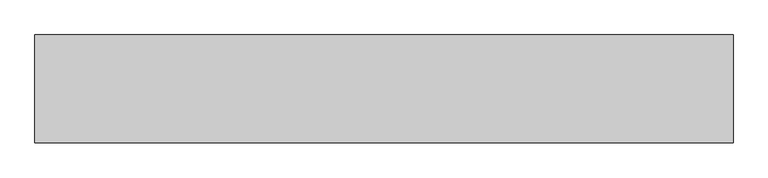
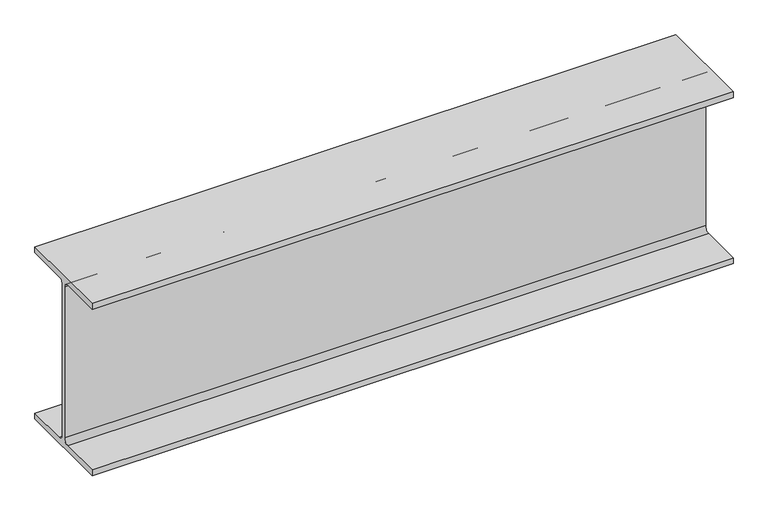
"""IFC4 building model written with IfcOpenShell, lengths in millimetres: beam geometry, Old_Steel Beam_H-KSD3502 : H_SB_ASB_H-194×150x6x9."""

import ifcopenshell
import ifcopenshell.guid

model = None  # the IFC model being written
_history = None  # IfcOwnerHistory: only IFC2X3 demands one
_inside = {}  # id of a spatial element -> (the spatial element, [elements in it])
_under = {}  # id of a project, library or spatial element -> (it, [spatial elements below it])
_declared = {}  # id of a project -> (the project, [libraries it declares])
_typed = {}  # id of a type object -> (the type object, [elements of that type])
_made_of = {}  # id of a material, layer set ... -> (it, [elements and type objects made of it])


def new_model(schema):
    """Start an empty IFC model of exactly this schema.

    Asked for "IFC4X3", IfcOpenShell would pick the latest addendum, in which some entities
    have other attributes; the version numbers below select the first issue.
    IFC2X3 requires an IfcOwnerHistory on every rooted entity: one is made here for all.
    """
    global model, _history
    if schema == "IFC4X3":
        model = ifcopenshell.file(schema_version=(4, 3, 0, 0))
    else:
        model = ifcopenshell.file(schema=schema)
    _inside.clear()
    _under.clear()
    _declared.clear()
    _typed.clear()
    _made_of.clear()
    _history = None
    if model.schema == "IFC2X3":
        org = make("IfcOrganization", Name="unknown")
        user = make(
            "IfcPersonAndOrganization",
            ThePerson=make("IfcPerson", FamilyName="unknown"),
            TheOrganization=org,
        )
        app = make(
            "IfcApplication",
            ApplicationDeveloper=org,
            Version="unknown",
            ApplicationFullName="unknown",
            ApplicationIdentifier="unknown",
        )
        _history = make(
            "IfcOwnerHistory",
            OwningUser=user,
            OwningApplication=app,
            ChangeAction="ADDED",
            CreationDate=0,
        )
    return model


def make(cls, **values):
    """One entity of the class cls with the attributes given. An attribute that is None is left unset."""
    return model.create_entity(
        cls, **{name: value for name, value in values.items() if value is not None}
    )


def rooted(cls, **values):
    """An entity with a GlobalId (a new one), such as an element, a storey or a relation."""
    return make(cls, GlobalId=ifcopenshell.guid.new(), OwnerHistory=_history, **values)


def si_unit(unit_type, name, prefix=None):
    """IfcSIUnit, for example si_unit("LENGTHUNIT", "METRE", prefix="MILLI")."""
    return make("IfcSIUnit", UnitType=unit_type, Prefix=prefix, Name=name)


def assignment(units):
    """IfcUnitAssignment: the units of a project."""
    return None if units is None else make("IfcUnitAssignment", Units=units)


def point(xyz):
    """IfcCartesianPoint."""
    return None if xyz is None else make("IfcCartesianPoint", Coordinates=xyz)


def direction(xyz):
    """IfcDirection."""
    return None if xyz is None else make("IfcDirection", DirectionRatios=xyz)


def frame(location, z_axis=None, x_axis=None):
    """IfcAxis2Placement3D, a coordinate frame: its origin and axes. An axis left out is left unset."""
    return make(
        "IfcAxis2Placement3D",
        Location=point(location),
        Axis=direction(z_axis),
        RefDirection=direction(x_axis),
    )


def frame_2d(location, x_axis=None):
    """IfcAxis2Placement2D, a coordinate frame in the plane: its origin and x axis."""
    return make(
        "IfcAxis2Placement2D", Location=point(location), RefDirection=direction(x_axis)
    )


def origin():
    """The frame at (0, 0, 0) with its axes left unset."""
    return frame((0.0, 0.0, 0.0))


def place(relative_to, where):
    """IfcLocalPlacement: puts the frame where relative to a parent placement (None: the world)."""
    return make(
        "IfcLocalPlacement", PlacementRelTo=relative_to, RelativePlacement=where
    )


def context(
    kind, dimensions, precision=None, world=None, true_north=None, identifier=None
):
    """IfcGeometricRepresentationContext, for example the 3D "Model" context."""
    return make(
        "IfcGeometricRepresentationContext",
        ContextIdentifier=identifier,
        ContextType=kind,
        CoordinateSpaceDimension=dimensions,
        Precision=precision,
        WorldCoordinateSystem=world,
        TrueNorth=true_north,
    )


def project(units=None, contexts=None):
    """IfcProject with its units and contexts."""
    return rooted(
        "IfcProject",
        Name="project",
        RepresentationContexts=contexts,
        UnitsInContext=assignment(units),
    )


def spatial(cls, under=None, at=None, **own):
    """A site, building, storey or space (cls), placed at a placement, below another one or the project."""
    s = rooted(cls, ObjectPlacement=at, **own)
    if under is not None:
        _under.setdefault(under.id(), (under, []))[1].append(s)
    return s


def polyline(points):
    """IfcPolyline through the points."""
    return make("IfcPolyline", Points=[point(p) for p in points])


def circle_curve(where, radius):
    """IfcCircle in the frame where."""
    return make("IfcCircle", Position=where, Radius=radius)


def trimmed(basis, trim1, trim2, sense, master):
    """IfcTrimmedCurve: the piece of a basis curve between two trims."""
    return make(
        "IfcTrimmedCurve",
        BasisCurve=basis,
        Trim1=trim1,
        Trim2=trim2,
        SenseAgreement=sense,
        MasterRepresentation=master,
    )


def segment(curve, same_sense, transition):
    """IfcCompositeCurveSegment."""
    return make(
        "IfcCompositeCurveSegment",
        Transition=transition,
        SameSense=same_sense,
        ParentCurve=curve,
    )


def composite_curve(segments, self_intersect=None):
    """IfcCompositeCurve: segments joined end to end."""
    return make("IfcCompositeCurve", Segments=segments, SelfIntersect=self_intersect)


def outline(outer, holes=None, kind="AREA"):
    """IfcArbitraryClosedProfileDef: a profile drawn as a closed curve; with holes, ...WithVoids."""
    if holes is None:
        return make("IfcArbitraryClosedProfileDef", ProfileType=kind, OuterCurve=outer)
    return make(
        "IfcArbitraryProfileDefWithVoids",
        ProfileType=kind,
        OuterCurve=outer,
        InnerCurves=holes,
    )


def extrude(swept, where, along, depth):
    """IfcExtrudedAreaSolid: the profile swept, set in the frame where, extruded along a direction by depth."""
    return make(
        "IfcExtrudedAreaSolid",
        SweptArea=swept,
        Position=where,
        ExtrudedDirection=direction(along),
        Depth=depth,
    )


def shape(context_of_items, identifier, shape_type, items):
    """IfcShapeRepresentation: the items that make up one representation, for example the "Body"."""
    return make(
        "IfcShapeRepresentation",
        ContextOfItems=context_of_items,
        RepresentationIdentifier=identifier,
        RepresentationType=shape_type,
        Items=items,
    )


def source(mapping_origin, context_of_items, identifier, shape_type, items):
    """IfcRepresentationMap: a shape defined once, which mapped items show again and again."""
    return make(
        "IfcRepresentationMap",
        MappingOrigin=mapping_origin,
        MappedRepresentation=shape(context_of_items, identifier, shape_type, items),
    )


def transform(
    local_origin,
    x_axis=None,
    y_axis=None,
    z_axis=None,
    scale=None,
    scale2=None,
    scale3=None,
    uniform=True,
):
    """IfcCartesianTransformationOperator3D, or its non-uniform kind. x_axis, y_axis, z_axis: its Axis1, 2, 3."""
    if uniform:
        return make(
            "IfcCartesianTransformationOperator3D",
            Axis1=direction(x_axis),
            Axis2=direction(y_axis),
            LocalOrigin=point(local_origin),
            Scale=scale,
            Axis3=direction(z_axis),
        )
    return make(
        "IfcCartesianTransformationOperator3DnonUniform",
        Axis1=direction(x_axis),
        Axis2=direction(y_axis),
        LocalOrigin=point(local_origin),
        Scale=scale,
        Axis3=direction(z_axis),
        Scale2=scale2,
        Scale3=scale3,
    )


def mapped(mapping_source, mapping_target):
    """IfcMappedItem: shows the shape of a source again, moved by a transform."""
    return make(
        "IfcMappedItem", MappingSource=mapping_source, MappingTarget=mapping_target
    )


def made_of(thing, what):
    """Note that an element or type object is made of a material, layer set ...; save() writes the relation."""
    if what is not None:
        _made_of.setdefault(what.id(), (what, []))[1].append(thing)
    return thing


def element(
    cls,
    number,
    at=None,
    inside=None,
    cuts=None,
    type_object=None,
    material=None,
    context=None,
    identifier="Body",
    shape_type=None,
    held_by="IfcProductDefinitionShape",
    body=None,
    shapes=None,
    **own,
):
    """One element of the class cls, such as IfcWall. Its Tag is "e" and its number.

    at: its placement. inside: the storey or other place that contains it. cuts: it is an
    opening in that element (IfcRelVoidsElement). A single representation is given by context,
    identifier, shape_type and body (its items); several are given by shapes. held_by: the class
    of the entity that holds the representations. save() writes the other relations.
    """
    e = rooted(cls, Tag="e%d" % number, ObjectPlacement=at, **own)
    if body is not None:
        shapes = [shape(context, identifier, shape_type, body)]
    if shapes is not None:
        e.Representation = make(held_by, Representations=shapes)
    if inside is not None:
        _inside.setdefault(inside.id(), (inside, []))[1].append(e)
    if cuts is not None:
        rooted(
            "IfcRelVoidsElement", RelatingBuildingElement=cuts, RelatedOpeningElement=e
        )
    if type_object is not None:
        _typed.setdefault(type_object.id(), (type_object, []))[1].append(e)
    return made_of(e, material)


def aggregate(whole, parts):
    """IfcRelAggregates: a whole, such as a stair, and the parts it consists of."""
    return rooted("IfcRelAggregates", RelatingObject=whole, RelatedObjects=parts)


def save(model, path):
    """Write the relations noted so far, then the file.

    IfcRelAggregates (storeys below a building ...), IfcRelContainedInSpatialStructure (elements
    in a storey), IfcRelDefinesByType, IfcRelAssociatesMaterial and IfcRelDeclares: one each for
    every whole, place, type object, material and project.
    """
    for whole, parts in _under.values():
        aggregate(whole, parts)
    for where, things in _inside.values():
        rooted(
            "IfcRelContainedInSpatialStructure",
            RelatedElements=things,
            RelatingStructure=where,
        )
    for kind, things in _typed.values():
        rooted("IfcRelDefinesByType", RelatedObjects=things, RelatingType=kind)
    for what, things in _made_of.values():
        rooted("IfcRelAssociatesMaterial", RelatedObjects=things, RelatingMaterial=what)
    for by, libraries in _declared.values():
        rooted("IfcRelDeclares", RelatingContext=by, RelatedDefinitions=libraries)
    model.write(path)


def beam_dbf2e1a8(model_context):
    return source(origin(), model_context, "Body", "SweptSolid", [
        extrude(outline(composite_curve([segment(polyline([(-82.5, -141.5), (-11.9, -141.5)]), True, "CONTINUOUS"), segment(trimmed(circle_curve(frame_2d((-11.9, -132.6)), 8.9), [point((-11.9, -141.5))], [point((-3.0, -132.6))], True, "CARTESIAN"), True, "CONTINUOUS"), segment(polyline([(-3.0, -132.6), (-3.0, 132.6)]), True, "CONTINUOUS"), segment(trimmed(circle_curve(frame_2d((-11.9, 132.6)), 8.9), [point((-3.0, 132.6))], [point((-11.9, 141.5))], True, "CARTESIAN"), True, "CONTINUOUS"), segment(polyline([(-11.9, 141.5), (-82.5, 141.5), (-82.5, 151.7), (82.5, 151.7), (82.5, 141.5), (11.9, 141.5)]), True, "CONTINUOUS"), segment(trimmed(circle_curve(frame_2d((11.9, 132.6)), 8.9), [point((11.9, 141.5))], [point((3.0, 132.6))], True, "CARTESIAN"), True, "CONTINUOUS"), segment(polyline([(3.0, 132.6), (3.0, -132.6)]), True, "CONTINUOUS"), segment(trimmed(circle_curve(frame_2d((11.9, -132.6)), 8.9), [point((3.0, -132.6))], [point((11.9, -141.5))], True, "CARTESIAN"), True, "CONTINUOUS"), segment(polyline([(11.9, -141.5), (82.5, -141.5), (82.5, -151.7), (-82.5, -151.7), (-82.5, -141.5)]), True, "CONTINUOUS")], self_intersect=False)), frame((-293.5180628, 0.0, 0.0), z_axis=(1.0, 0.0, 0.0), x_axis=(0.0, 1.0, 0.0)), (0.0, 0.0, 1.0), 1068.0320464),
    ])


if __name__ == "__main__":
    model = new_model("IFC4")
    model_context = context("Model", 3, world=origin())
    ifc_project = project(units=[si_unit("LENGTHUNIT", "METRE", prefix="MILLI")], contexts=[model_context])
    site = spatial("IfcSite", under=ifc_project)
    building = spatial("IfcBuilding", under=site)
    placement = place(None, origin())
    beam_shape = beam_dbf2e1a8(model_context)
    element("IfcBeam", 1, ObjectType="Old_Steel Beam_H-KSD3502 : H_SB_ASB_H-194×150x6x9", at=placement, inside=building, context=model_context, shape_type="MappedRepresentation", body=[
        mapped(beam_shape, transform((0.0, 0.0, 0.0), x_axis=(1.0, 0.0, 0.0), y_axis=(0.0, 1.0, 0.0), z_axis=(0.0, 0.0, 1.0))),
    ])
    save(model, "model.ifc")

# Revit data of these elements
# Type "Old_Steel Beam_H-KSD3502 : H_SB_ASB_H-194×150x6x9"
#   Width = 15.0 cm
#   Web Thickness = 0.6 cm
#   Web Fillet = 1.3 cm
#   Warping Constant = 43316.0 cm⁶
#   Torsional Moment of Inertia = 8.622 cm⁴
#   Torsional Modulus = 1.0 cm³
#   Section Area = 39.01 cm²
#   Plastic Modulus weak axis = 104.0 cm³
#   Plastic Modulus strong axis = 309.0 cm³
#   Perimeter = 0.95 m²/m
#   Nominal Weight = 30.60 kgf/m
#   Moment of Inertia weak axis = 507.00 cm⁴
#   Moment of Inertia strong axis = 2690.00 cm⁴
#   Height = 19.4 cm
#   Flange Thickness = 0.9 cm
#   Elastic Modulus weak axis = 67.6 cm³
#   Elastic Modulus strong axis = 277.0 cm³
#   Centroid Vertical = 9.7 cm
#   Centroid Horizontal = 7.5 cm
#   Length [instance default] = 1.5240 m
#   Structural Material [instance default] = Steel, 45-345
#   Assembly Code = ""
# Element 1 (IfcBeam, "Old_Steel Beam_H-KSD3502 : H_SB_ASB_H-194×150x6x9")
#   Structural Material = none
# Materials
#   "Steel, 45-345": class "Metal", colour RGB 189 187 185, transparency 0, Description = "Steel 345 MPa", Cost = 0
